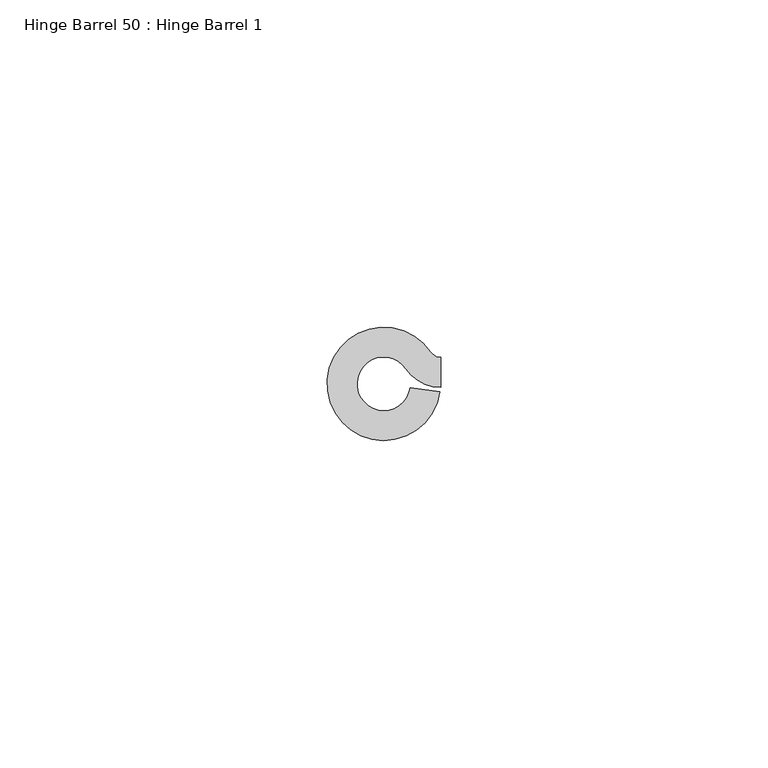
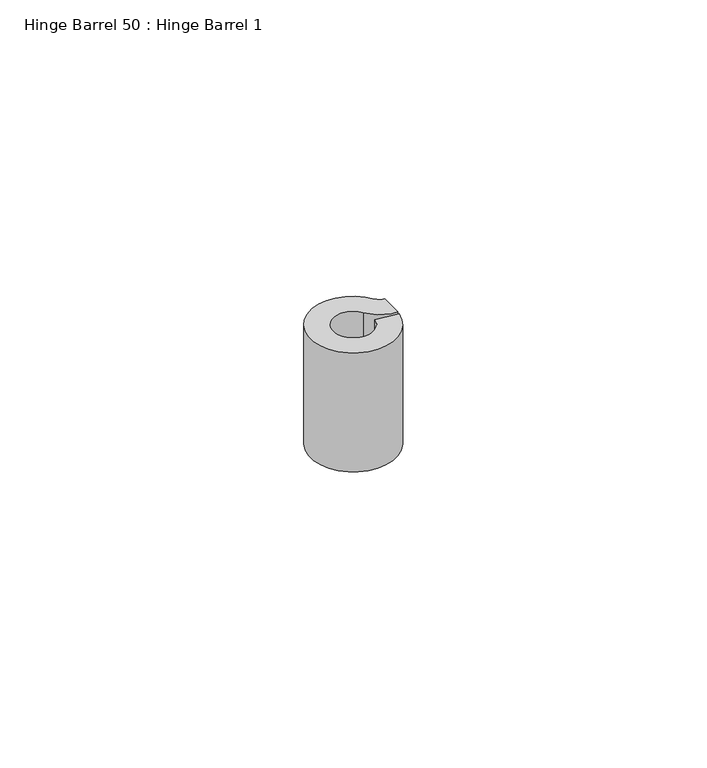
"""IFC4 building model written with IfcOpenShell, lengths in millimetres: proxy geometry, Hinge Barrel 50 : Hinge Barrel 1."""

from ifc_helpers import new_model, si_unit, point, frame, frame_2d, origin, place, context, project, spatial, polyline, circle_curve, trimmed, segment, composite_curve, outline, extrude, source, transform, mapped, element, save


def hinge_barrel_50_hinge_barrel_1_a09c7832(model_context):
    return source(origin(), model_context, "Body", "SweptSolid", [
        extrude(outline(composite_curve([segment(trimmed(circle_curve(frame_2d((587319.1320739, -534100.7049841)), 4.0894), [point((587322.5194669, -534098.4139665))], [point((587323.1821338, -534101.2708529))], True, "CARTESIAN"), True, "CONTINUOUS"), segment(polyline([(587323.1821338, -534101.2708529), (587327.7022899, -534101.9024028)]), True, "CONTINUOUS"), segment(trimmed(circle_curve(frame_2d((587319.1320739, -534100.7049841)), 8.6534625), [point((587327.7022899, -534101.9024028))], [point((587326.3000393, -534095.8570273))], False, "CARTESIAN"), True, "CONTINUOUS"), segment(trimmed(circle_curve(frame_2d((587327.8245257, -534094.8259615)), 1.8404226), [point((587326.3000393, -534095.8570273))], [point((587327.8245257, -534096.6663841))], True, "CARTESIAN"), True, "CONTINUOUS"), segment(polyline([(587327.8245257, -534096.6663841), (587327.8245257, -534101.2304466)]), True, "CONTINUOUS"), segment(trimmed(circle_curve(frame_2d((587327.8245257, -534094.8259615)), 6.4044851), [point((587327.8245257, -534101.2304466))], [point((587322.5194669, -534098.4139665))], False, "CARTESIAN"), True, "CONTINUOUS")], self_intersect=False)), frame((0.0, 0.0, 1149.35), z_axis=(0.0, 0.0, 1.0), x_axis=(1.0, 0.0, 0.0)), (0.0, 0.0, 1.0), 25.4),
    ])


if __name__ == "__main__":
    model = new_model("IFC4")
    model_context = context("Model", 3, world=origin())
    ifc_project = project(units=[si_unit("LENGTHUNIT", "METRE", prefix="MILLI")], contexts=[model_context])
    site = spatial("IfcSite", under=ifc_project)
    building = spatial("IfcBuilding", under=site)
    placement = place(None, origin())
    hinge_barrel_50_hinge_barrel_1_shape = hinge_barrel_50_hinge_barrel_1_a09c7832(model_context)
    element("IfcBuildingElementProxy", 1, Name="Hinge Barrel 50 : Hinge Barrel 1", ObjectType="Hinge Barrel 50 : Hinge Barrel 1", at=placement, inside=building, context=model_context, shape_type="MappedRepresentation", body=[
        mapped(hinge_barrel_50_hinge_barrel_1_shape, transform((0.0, 0.0, 0.0), x_axis=(1.0, 0.0, 0.0), y_axis=(0.0, 1.0, 0.0), z_axis=(0.0, 0.0, 1.0))),
    ])
    save(model, "model.ifc")

# Revit data of these elements
# Element 1 (IfcBuildingElementProxy, "Hinge Barrel 50 : Hinge Barrel 1")
#   Materials on its faces: "6\"X6\" WELD-ON STL BUTT HINGE"
# Materials
#   "6\"X6\" WELD-ON STL BUTT HINGE": class "Metal", colour RGB 189 187 185, transparency 0, Description = "Carbon steel", Cost = 0
